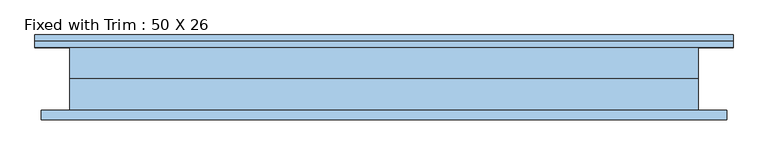
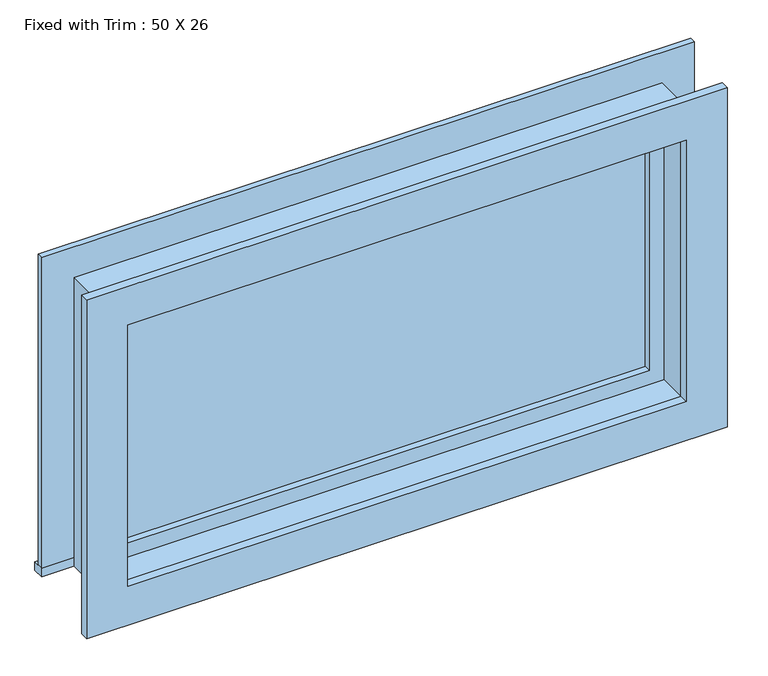
"""IFC4 building model written with IfcOpenShell, lengths in millimetres: window geometry, Fixed with Trim : 50 X 26."""

from ifc_helpers import new_model, si_unit, frame, origin, place, context, project, spatial, polyline, outline, extrude, source, transform, mapped, element, save


def fixed_with_trim_50_x_26_c3637fcc(model_context):
    return source(origin(), model_context, "Body", "SweptSolid", [
        extrude(outline(polyline([(-742.95, 88.9), (666.75, 88.9), (666.75, 63.5), (-742.95, 63.5), (-742.95, 88.9)])), frame((0.0, 0.0, 914.4), z_axis=(0.0, 0.0, 1.0), x_axis=(1.0, 0.0, 0.0)), (0.0, 0.0, 1.0), 19.05),
        extrude(outline(polyline([(1555.75, -654.05), (1555.75, 577.85), (933.45, 577.85), (933.45, 666.75), (1644.65, 666.75), (1644.65, -742.95), (933.45, -742.95), (933.45, -654.05), (1555.75, -654.05)])), frame((0.0, 63.5, 0.0), z_axis=(0.0, 1.0, 0.0), x_axis=(0.0, 0.0, 1.0)), (0.0, 0.0, 1.0), 12.7),
        extrude(outline(polyline([(1631.95, 654.05), (1631.95, -730.25), (857.25, -730.25), (857.25, 654.05), (1631.95, 654.05)]), holes=[polyline([(1543.05, 565.15), (946.15, 565.15), (946.15, -641.35), (1543.05, -641.35), (1543.05, 565.15)])]), frame((0.0, -82.55, 0.0), z_axis=(0.0, 1.0, 0.0), x_axis=(0.0, 0.0, 1.0)), (0.0, 0.0, 1.0), 19.05),
        extrude(outline(polyline([(533.4, 15.875), (-609.6, 15.875), (-609.6, 28.575), (533.4, 28.575), (533.4, 15.875)])), frame((0.0, 0.0, 977.9), z_axis=(0.0, 0.0, 1.0), x_axis=(1.0, 0.0, 0.0)), (0.0, 0.0, 1.0), 533.4),
        extrude(outline(polyline([(1555.75, -654.05), (933.45, -654.05), (933.45, 577.85), (1555.75, 577.85), (1555.75, -654.05)]), holes=[polyline([(1511.3, -609.6), (1511.3, 533.4), (977.9, 533.4), (977.9, -609.6), (1511.3, -609.6)])]), frame((0.0, 0.0, 0.0), z_axis=(0.0, 1.0, 0.0), x_axis=(0.0, 0.0, 1.0)), (0.0, 0.0, 1.0), 44.45),
        extrude(outline(polyline([(1574.8, -673.1), (914.4, -673.1), (914.4, 596.9), (1574.8, 596.9), (1574.8, -673.1)]), holes=[polyline([(1543.05, -641.35), (1543.05, 565.15), (946.15, 565.15), (946.15, -641.35), (1543.05, -641.35)])]), frame((0.0, -63.5, 0.0), z_axis=(0.0, 1.0, 0.0), x_axis=(0.0, 0.0, 1.0)), (0.0, 0.0, 1.0), 63.5),
        extrude(outline(polyline([(1574.8, 596.9), (1574.8, -673.1), (914.4, -673.1), (914.4, 596.9), (1574.8, 596.9)]), holes=[polyline([(1555.75, 577.85), (933.45, 577.85), (933.45, -654.05), (1555.75, -654.05), (1555.75, 577.85)])]), frame((0.0, 0.0, 0.0), z_axis=(0.0, 1.0, 0.0), x_axis=(0.0, 0.0, 1.0)), (0.0, 0.0, 1.0), 63.5),
    ])


if __name__ == "__main__":
    model = new_model("IFC4")
    model_context = context("Model", 3, world=origin())
    ifc_project = project(units=[si_unit("LENGTHUNIT", "METRE", prefix="MILLI")], contexts=[model_context])
    site = spatial("IfcSite", under=ifc_project)
    building = spatial("IfcBuilding", under=site)
    placement = place(None, origin())
    fixed_with_trim_50_x_26_shape = fixed_with_trim_50_x_26_c3637fcc(model_context)
    element("IfcWindow", 1, ObjectType="Fixed with Trim : 50 X 26", at=placement, inside=building, context=model_context, shape_type="MappedRepresentation", body=[
        mapped(fixed_with_trim_50_x_26_shape, transform((0.0, 0.0, 0.0), x_axis=(1.0, 0.0, 0.0), y_axis=(0.0, 1.0, 0.0), z_axis=(0.0, 0.0, 1.0))),
    ])
    save(model, "model.ifc")

# Revit data of these elements
# Type "Fixed with Trim : 50 X 26"
#   Type Mark = "62"
#   Construction Type Id = "GSP4R"
#   Assembly Code = "B2020100"
#   Analytic Construction = "1/8 in Pilkington single glazing"
#   Visual Light Transmittance = 0.9
#   Solar Heat Gain Coefficient = 0.78
#   Heat Transfer Coefficient (U) = 3.6886 W/(m²·K)
#   Height = 2' - 2"
#   Default Sill Height = 3' - 0"
#   Trim Projection - Ext. = 0' - 0 1/2"
#   Trim Projection - Int. = 0' - 0 3/4"
#   Trim Width - Exterior = 0' - 3 1/2"
#   Trim Width - Interior = 0' - 3 1/2"
#   Width = 4' - 2"
#   Window Inset = 0' - 0 3/4"
#   Glass Pane Material = EXISTING WINDOW
#   Sash Material = Trim
#   Trim Exterior Material = Trim
#   Trim Interior Material = Trim
#   Wall Closure = (empty or 0)
# Element 1 (IfcWindow, "Fixed with Trim : 50 X 26")
#   Materials on its faces: "Trim", "EXISTING WINDOW"
# Materials
#   "EXISTING WINDOW": class "Glass", colour RGB 218 227 224, transparency 0.85, Description = "Soda Lime Glass", Cost = 0
#   "Trim": class "Wood", colour RGB 250 251 245, transparency 0, Cost = 0
